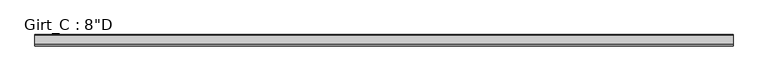
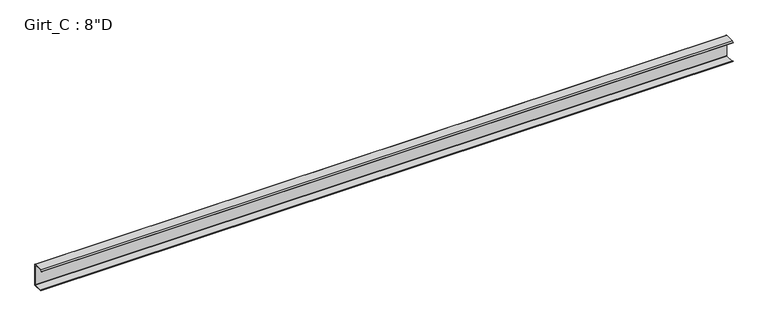
"""IFC4 building model written with IfcOpenShell, lengths in millimetres: beam geometry."""

from ifc_helpers import new_model, si_unit, point, frame, frame_2d, origin, place, context, project, spatial, polyline, circle_curve, trimmed, segment, composite_curve, outline, extrude, source, transform, mapped, element, save


def beam_9dc17019(model_context):
    return source(origin(), model_context, "Body", "SweptSolid", [
        extrude(outline(composite_curve([segment(polyline([(-87.5109375, 101.6), (-3.3734375, 101.6)]), True, "CONTINUOUS"), segment(trimmed(circle_curve(frame_2d((-3.3734375, 96.8375)), 4.7625), [point((-3.3734375, 101.6))], [point((1.3890625, 96.8375))], False, "CARTESIAN"), True, "CONTINUOUS"), segment(polyline([(1.3890625, 96.8375), (1.3890625, -96.8375)]), True, "CONTINUOUS"), segment(trimmed(circle_curve(frame_2d((-3.3734375, -96.8375)), 4.7625), [point((1.3890625, -96.8375))], [point((-3.3734375, -101.6))], False, "CARTESIAN"), True, "CONTINUOUS"), segment(polyline([(-3.3734375, -101.6), (-87.5109375, -101.6), (-99.7792647, -86.979177), (-97.6510975, -85.1934327), (-86.2154765, -98.821875), (-3.2694106, -98.821875)]), True, "CONTINUOUS"), segment(trimmed(circle_curve(frame_2d((-3.3748024, -96.8389339)), 1.9857399), [point((-3.2694106, -98.821875))], [point((-1.3890625, -96.8389339))], True, "CARTESIAN"), True, "CONTINUOUS"), segment(polyline([(-1.3890625, -96.8389339), (-1.3890625, 96.8381931)]), True, "CONTINUOUS"), segment(trimmed(circle_curve(frame_2d((-3.3741066, 96.8381931)), 1.9850441), [point((-1.3890625, 96.8381931))], [point((-3.3005807, 98.821875))], True, "CARTESIAN"), True, "CONTINUOUS"), segment(polyline([(-3.3005807, 98.821875), (-86.2154765, 98.821875), (-97.6278742, 85.221109), (-99.7560415, 87.0068534), (-87.5109375, 101.6)]), True, "CONTINUOUS")], self_intersect=False)), frame((-3067.9362419, 0.0, 0.0), z_axis=(1.0, 0.0, 0.0), x_axis=(0.0, 1.0, 0.0)), (0.0, 0.0, 1.0), 6251.575),
    ])


if __name__ == "__main__":
    model = new_model("IFC4")
    model_context = context("Model", 3, world=origin())
    ifc_project = project(units=[si_unit("LENGTHUNIT", "METRE", prefix="MILLI")], contexts=[model_context])
    site = spatial("IfcSite", under=ifc_project)
    building = spatial("IfcBuilding", under=site)
    placement = place(None, origin())
    beam_shape = beam_9dc17019(model_context)
    element("IfcBeam", 1, ObjectType="Girt_C : 8\"D", at=placement, inside=building, context=model_context, shape_type="MappedRepresentation", body=[
        mapped(beam_shape, transform((0.0, 0.0, 0.0), x_axis=(1.0, 0.0, 0.0), y_axis=(0.0, 1.0, 0.0), z_axis=(0.0, 0.0, 1.0))),
    ])
    save(model, "model.ifc")

# Revit data of these elements
# Type "Girt_C : 8\"D"
#   half leg = 0' - 1 3/4"
#   Web_Thickness = 0' - 0 7/64"
#   Length [instance default] = 10' - 0"
#   Leg_1 = 0' - 3 1/2"
#   Height = 0' - 8"
#   Structural Material [instance default] = none
# Element 1 (IfcBeam, "Girt_C : 8\"D")
#   Structural Material = GALVANIZED 'CEE' SECTION (8.0x3.5C - SEE STRUCT. DWGS)
#   Materials on its faces: "GALVANIZED 'CEE' SECTION (8.0x3.5C - SEE STRUCT. DWGS)"
# Materials
#   "GALVANIZED 'CEE' SECTION (8.0x3.5C - SEE STRUCT. DWGS)": class "Metal", colour RGB 137 146 153, transparency 0, Description = "Steel, mill finish", Cost = 0
